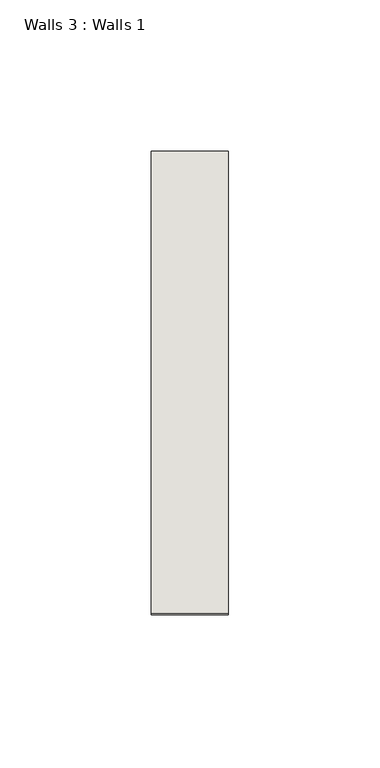
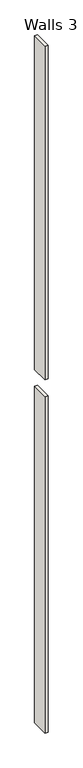
"""IFC4 building model written with IfcOpenShell, lengths in millimetres: wall geometry, Walls 3 : Walls 1."""

from ifc_helpers import new_model, si_unit, frame, origin, origin_with_axes, place, context, project, spatial, polyline, outline, extrude, source, transform, mapped, element, save


def walls_3_walls_1_bbe09ba3(model_context):
    return source(origin(), model_context, "Body", "SweptSolid", [
        extrude(outline(polyline([(25761.6402986, -14033.9330088), (25787.0402986, -14033.9330088), (25787.0402986, -14186.3330088), (25761.6402986, -14186.3330088), (25761.6402986, -14033.9330088)])), frame((0.0, 0.0, 3200.4), z_axis=(0.0, 0.0, 1.0), x_axis=(1.0, 0.0, 0.0)), (0.0, 0.0, 1.0), 3022.6),
        extrude(outline(polyline([(25787.0402986, -14033.9330088), (25787.0402986, -14186.3330088), (25761.6402986, -14186.3330088), (25761.6402986, -14033.9330088), (25787.0402986, -14033.9330088)])), origin_with_axes(), (0.0, 0.0, 1.0), 3048.0),
    ])


if __name__ == "__main__":
    model = new_model("IFC4")
    model_context = context("Model", 3, world=origin())
    ifc_project = project(units=[si_unit("LENGTHUNIT", "METRE", prefix="MILLI")], contexts=[model_context])
    site = spatial("IfcSite", under=ifc_project)
    building = spatial("IfcBuilding", under=site)
    placement = place(None, origin())
    walls_3_walls_1_shape = walls_3_walls_1_bbe09ba3(model_context)
    element("IfcWall", 1, ObjectType="Walls 3 : Walls 1", at=placement, inside=building, context=model_context, shape_type="MappedRepresentation", body=[
        mapped(walls_3_walls_1_shape, transform((0.0, 0.0, 0.0), x_axis=(1.0, 0.0, 0.0), y_axis=(0.0, 1.0, 0.0), z_axis=(0.0, 0.0, 1.0))),
    ])
    save(model, "model.ifc")

# Revit data of these elements
# Element 1 (IfcWall, "Walls 3 : Walls 1")
#   Materials on its faces: "Trim", "WHITE PAINT ON WOOD"
# Materials
#   "Trim": class "Wood", colour RGB 250 251 245, transparency 0, Cost = 0
#   "WHITE PAINT ON WOOD": class "Paint", colour RGB 255 255 255, transparency 0, Cost = 0
